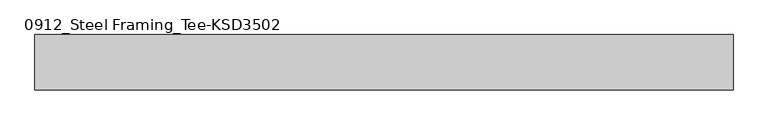
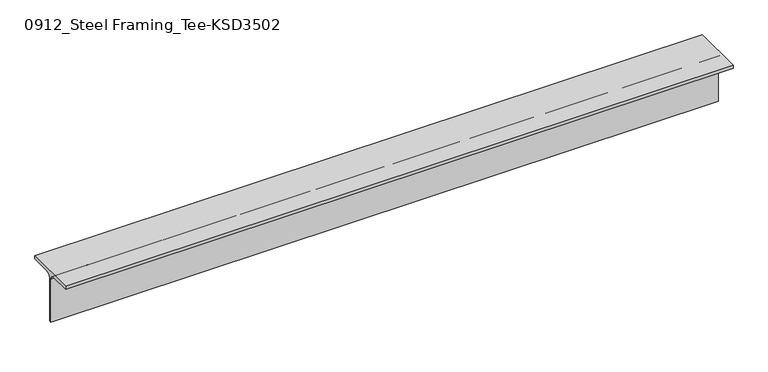
"""IFC4 building model written with IfcOpenShell, lengths in millimetres: member geometry, 0912_Steel Framing_Tee-KSD3502 : H_SB_ASB_CT-150x150x6.5x9."""

from ifc_helpers import new_model, si_unit, point, frame, frame_2d, origin, place, context, project, spatial, polyline, circle_curve, trimmed, segment, composite_curve, outline, extrude, source, transform, mapped, element, save


def member_0912_steel_framing_tee_ksd3502_efa4219b(model_context):
    return source(origin(), model_context, "Body", "SweptSolid", [
        extrude(outline(composite_curve([segment(polyline([(75.0, 75.0), (75.0, 66.0), (16.25, 66.0)]), True, "CONTINUOUS"), segment(trimmed(circle_curve(frame_2d((16.25, 53.0)), 13.0), [point((16.25, 66.0))], [point((3.25, 53.0))], True, "CARTESIAN"), True, "CONTINUOUS"), segment(polyline([(3.25, 53.0), (3.25, -75.0), (-3.25, -75.0), (-3.25, 53.0)]), True, "CONTINUOUS"), segment(trimmed(circle_curve(frame_2d((-16.25, 53.0)), 13.0), [point((-3.25, 53.0))], [point((-16.25, 66.0))], True, "CARTESIAN"), True, "CONTINUOUS"), segment(polyline([(-16.25, 66.0), (-75.0, 66.0), (-75.0, 75.0), (75.0, 75.0)]), True, "CONTINUOUS")], self_intersect=False)), frame((-983.95, 0.0, 0.0), z_axis=(1.0, 0.0, 0.0), x_axis=(0.0, 1.0, 0.0)), (0.0, 0.0, 1.0), 1884.0),
    ])


if __name__ == "__main__":
    model = new_model("IFC4")
    model_context = context("Model", 3, world=origin())
    ifc_project = project(units=[si_unit("LENGTHUNIT", "METRE", prefix="MILLI")], contexts=[model_context])
    site = spatial("IfcSite", under=ifc_project)
    building = spatial("IfcBuilding", under=site)
    placement = place(None, origin())
    member_0912_steel_framing_tee_ksd3502_shape = member_0912_steel_framing_tee_ksd3502_efa4219b(model_context)
    element("IfcMember", 1, ObjectType="0912_Steel Framing_Tee-KSD3502 : H_SB_ASB_CT-150x150x6.5x9", at=placement, inside=building, context=model_context, shape_type="MappedRepresentation", body=[
        mapped(member_0912_steel_framing_tee_ksd3502_shape, transform((0.0, 0.0, 0.0), x_axis=(1.0, 0.0, 0.0), y_axis=(0.0, 1.0, 0.0), z_axis=(0.0, 0.0, 1.0))),
    ])
    save(model, "model.ifc")

# Revit data of these elements
# Type "0912_Steel Framing_Tee-KSD3502 : H_SB_ASB_CT-150x150x6.5x9"
#   H_WM Code_1 = "S01AA003-00001 | Main Steel Structure Fabrication Work | Shelter/Building | Light Steel - Standard (30KG/M>Weight) | Material: (   )"
#   H_WM Code_2 = "S03AA029-00001 | Main Steel Structure Erection Work | Shelter/Building | Light Steel (30KG/M>Weight) | Material: (   )"
#   H_WM Code_3 = "S01AA010-00001 | Main Steel Structure Fabrication Work | Shelter/Building | Steel Painting/Coating | for Non-Fireproofed Steel Surface, Surface Preparation, Primer, Second & Final Coat | Material: (   )"
#   H_Q'ty Cal Type Tag = "SB-Q2"
#   Width = 15.0 cm
#   Web Thickness = 0.65 cm
#   Web Fillet = 1.3 cm
#   Section Area = 23.39 cm²
#   Perimeter = 0.60 m²/m
#   Nominal Weight = 18.40 kgf/m
#   Height = 15.0 cm
#   Flange Thickness = 0.9 cm
#   Centroid Vertical = 7.5 cm
#   Centroid Horizontal = 7.5 cm
#   Length [instance default] = 1.5000 m
#   Structural Material [instance default] = Steel, 45-345
#   Warping Constant = (empty or 0)
#   Torsional Moment of Inertia = 0
#   Section Name Key = ""
#   Plastic Modulus weak axis = 0
#   Plastic Modulus strong axis = 0
#   Moment of Inertia weak axis = 0
#   Moment of Inertia strong axis = 0
#   Elastic Modulus weak axis = 0
#   Elastic Modulus strong axis = 0
#   Bolt Spacing = 0
#   Assembly Code = ""
# Element 1 (IfcMember, "0912_Steel Framing_Tee-KSD3502 : H_SB_ASB_CT-150x150x6.5x9")
#   Structural Material = none
# Materials
#   "Steel, 45-345": class "Metal", colour RGB 189 187 185, transparency 0, Description = "Steel 345 MPa", Cost = 0
